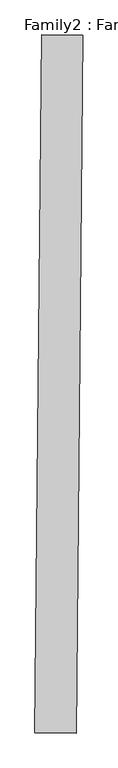
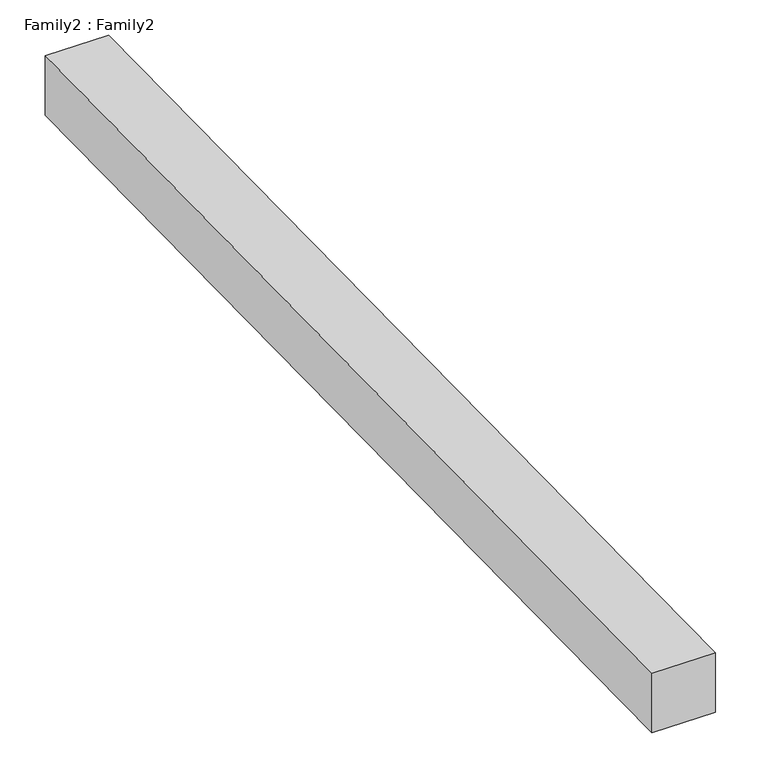
"""IFC4 building model written with IfcOpenShell, lengths in millimetres: proxy geometry, Family2 : Family2."""

from ifc_helpers import new_model, si_unit, origin, place, context, project, spatial, faceted_brep, source, transform, mapped, element, save


def family2_family2_2285597e(model_context):
    return source(origin(), model_context, "Body", "Brep", [
        faceted_brep([(-3960.1613892, -7770.4345052, 1.0945136), (-3960.1613892, -7770.4345052, 201.0945136), (-3926.6814053, -4377.1656174, 202.060409), (-3926.6814053, -4377.1656174, 2.060409), (-3760.1701992, -7772.3117178, 201.0945136), (-3726.6902153, -4379.0428301, 202.060409), (-3760.1701992, -7772.3117178, 1.0945136), (-3726.6902153, -4379.0428301, 2.060409)], [[[0, 1, 2, 3]], [[1, 4, 5, 2]], [[4, 6, 7, 5]], [[6, 0, 3, 7]], [[3, 2, 5, 7]], [[0, 6, 4, 1]]]),
    ])


if __name__ == "__main__":
    model = new_model("IFC4")
    model_context = context("Model", 3, world=origin())
    ifc_project = project(units=[si_unit("LENGTHUNIT", "METRE", prefix="MILLI")], contexts=[model_context])
    site = spatial("IfcSite", under=ifc_project)
    building = spatial("IfcBuilding", under=site)
    placement = place(None, origin())
    family2_family2_shape = family2_family2_2285597e(model_context)
    element("IfcBuildingElementProxy", 1, Name="Family2 : Family2", ObjectType="Family2 : Family2", at=placement, inside=building, context=model_context, shape_type="MappedRepresentation", body=[
        mapped(family2_family2_shape, transform((0.0, 0.0, 0.0), x_axis=(1.0, 0.0, 0.0), y_axis=(0.0, 1.0, 0.0), z_axis=(0.0, 0.0, 1.0))),
    ])
    save(model, "model.ifc")

# Revit data of these elements
# Type "Family2 : Family2"
#   Default Elevation = 0
